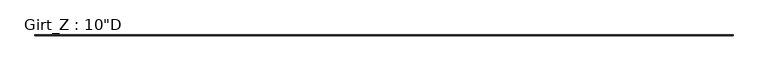
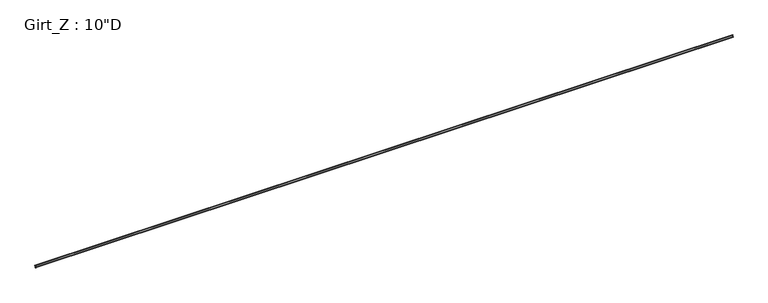
"""IFC4 building model written with IfcOpenShell, lengths in millimetres: beam geometry."""

import ifcopenshell
import ifcopenshell.guid

model = None  # the IFC model being written
_history = None  # IfcOwnerHistory: only IFC2X3 demands one
_inside = {}  # id of a spatial element -> (the spatial element, [elements in it])
_under = {}  # id of a project, library or spatial element -> (it, [spatial elements below it])
_declared = {}  # id of a project -> (the project, [libraries it declares])
_typed = {}  # id of a type object -> (the type object, [elements of that type])
_made_of = {}  # id of a material, layer set ... -> (it, [elements and type objects made of it])


def new_model(schema):
    """Start an empty IFC model of exactly this schema.

    Asked for "IFC4X3", IfcOpenShell would pick the latest addendum, in which some entities
    have other attributes; the version numbers below select the first issue.
    IFC2X3 requires an IfcOwnerHistory on every rooted entity: one is made here for all.
    """
    global model, _history
    if schema == "IFC4X3":
        model = ifcopenshell.file(schema_version=(4, 3, 0, 0))
    else:
        model = ifcopenshell.file(schema=schema)
    _inside.clear()
    _under.clear()
    _declared.clear()
    _typed.clear()
    _made_of.clear()
    _history = None
    if model.schema == "IFC2X3":
        org = make("IfcOrganization", Name="unknown")
        user = make(
            "IfcPersonAndOrganization",
            ThePerson=make("IfcPerson", FamilyName="unknown"),
            TheOrganization=org,
        )
        app = make(
            "IfcApplication",
            ApplicationDeveloper=org,
            Version="unknown",
            ApplicationFullName="unknown",
            ApplicationIdentifier="unknown",
        )
        _history = make(
            "IfcOwnerHistory",
            OwningUser=user,
            OwningApplication=app,
            ChangeAction="ADDED",
            CreationDate=0,
        )
    return model


def make(cls, **values):
    """One entity of the class cls with the attributes given. An attribute that is None is left unset."""
    return model.create_entity(
        cls, **{name: value for name, value in values.items() if value is not None}
    )


def rooted(cls, **values):
    """An entity with a GlobalId (a new one), such as an element, a storey or a relation."""
    return make(cls, GlobalId=ifcopenshell.guid.new(), OwnerHistory=_history, **values)


def si_unit(unit_type, name, prefix=None):
    """IfcSIUnit, for example si_unit("LENGTHUNIT", "METRE", prefix="MILLI")."""
    return make("IfcSIUnit", UnitType=unit_type, Prefix=prefix, Name=name)


def assignment(units):
    """IfcUnitAssignment: the units of a project."""
    return None if units is None else make("IfcUnitAssignment", Units=units)


def point(xyz):
    """IfcCartesianPoint."""
    return None if xyz is None else make("IfcCartesianPoint", Coordinates=xyz)


def direction(xyz):
    """IfcDirection."""
    return None if xyz is None else make("IfcDirection", DirectionRatios=xyz)


def frame(location, z_axis=None, x_axis=None):
    """IfcAxis2Placement3D, a coordinate frame: its origin and axes. An axis left out is left unset."""
    return make(
        "IfcAxis2Placement3D",
        Location=point(location),
        Axis=direction(z_axis),
        RefDirection=direction(x_axis),
    )


def frame_2d(location, x_axis=None):
    """IfcAxis2Placement2D, a coordinate frame in the plane: its origin and x axis."""
    return make(
        "IfcAxis2Placement2D", Location=point(location), RefDirection=direction(x_axis)
    )


def origin():
    """The frame at (0, 0, 0) with its axes left unset."""
    return frame((0.0, 0.0, 0.0))


def place(relative_to, where):
    """IfcLocalPlacement: puts the frame where relative to a parent placement (None: the world)."""
    return make(
        "IfcLocalPlacement", PlacementRelTo=relative_to, RelativePlacement=where
    )


def context(
    kind, dimensions, precision=None, world=None, true_north=None, identifier=None
):
    """IfcGeometricRepresentationContext, for example the 3D "Model" context."""
    return make(
        "IfcGeometricRepresentationContext",
        ContextIdentifier=identifier,
        ContextType=kind,
        CoordinateSpaceDimension=dimensions,
        Precision=precision,
        WorldCoordinateSystem=world,
        TrueNorth=true_north,
    )


def project(units=None, contexts=None):
    """IfcProject with its units and contexts."""
    return rooted(
        "IfcProject",
        Name="project",
        RepresentationContexts=contexts,
        UnitsInContext=assignment(units),
    )


def spatial(cls, under=None, at=None, **own):
    """A site, building, storey or space (cls), placed at a placement, below another one or the project."""
    s = rooted(cls, ObjectPlacement=at, **own)
    if under is not None:
        _under.setdefault(under.id(), (under, []))[1].append(s)
    return s


def polyline(points):
    """IfcPolyline through the points."""
    return make("IfcPolyline", Points=[point(p) for p in points])


def circle_curve(where, radius):
    """IfcCircle in the frame where."""
    return make("IfcCircle", Position=where, Radius=radius)


def trimmed(basis, trim1, trim2, sense, master):
    """IfcTrimmedCurve: the piece of a basis curve between two trims."""
    return make(
        "IfcTrimmedCurve",
        BasisCurve=basis,
        Trim1=trim1,
        Trim2=trim2,
        SenseAgreement=sense,
        MasterRepresentation=master,
    )


def segment(curve, same_sense, transition):
    """IfcCompositeCurveSegment."""
    return make(
        "IfcCompositeCurveSegment",
        Transition=transition,
        SameSense=same_sense,
        ParentCurve=curve,
    )


def composite_curve(segments, self_intersect=None):
    """IfcCompositeCurve: segments joined end to end."""
    return make("IfcCompositeCurve", Segments=segments, SelfIntersect=self_intersect)


def outline(outer, holes=None, kind="AREA"):
    """IfcArbitraryClosedProfileDef: a profile drawn as a closed curve; with holes, ...WithVoids."""
    if holes is None:
        return make("IfcArbitraryClosedProfileDef", ProfileType=kind, OuterCurve=outer)
    return make(
        "IfcArbitraryProfileDefWithVoids",
        ProfileType=kind,
        OuterCurve=outer,
        InnerCurves=holes,
    )


def extrude(swept, where, along, depth):
    """IfcExtrudedAreaSolid: the profile swept, set in the frame where, extruded along a direction by depth."""
    return make(
        "IfcExtrudedAreaSolid",
        SweptArea=swept,
        Position=where,
        ExtrudedDirection=direction(along),
        Depth=depth,
    )


def shape(context_of_items, identifier, shape_type, items):
    """IfcShapeRepresentation: the items that make up one representation, for example the "Body"."""
    return make(
        "IfcShapeRepresentation",
        ContextOfItems=context_of_items,
        RepresentationIdentifier=identifier,
        RepresentationType=shape_type,
        Items=items,
    )


def source(mapping_origin, context_of_items, identifier, shape_type, items):
    """IfcRepresentationMap: a shape defined once, which mapped items show again and again."""
    return make(
        "IfcRepresentationMap",
        MappingOrigin=mapping_origin,
        MappedRepresentation=shape(context_of_items, identifier, shape_type, items),
    )


def transform(
    local_origin,
    x_axis=None,
    y_axis=None,
    z_axis=None,
    scale=None,
    scale2=None,
    scale3=None,
    uniform=True,
):
    """IfcCartesianTransformationOperator3D, or its non-uniform kind. x_axis, y_axis, z_axis: its Axis1, 2, 3."""
    if uniform:
        return make(
            "IfcCartesianTransformationOperator3D",
            Axis1=direction(x_axis),
            Axis2=direction(y_axis),
            LocalOrigin=point(local_origin),
            Scale=scale,
            Axis3=direction(z_axis),
        )
    return make(
        "IfcCartesianTransformationOperator3DnonUniform",
        Axis1=direction(x_axis),
        Axis2=direction(y_axis),
        LocalOrigin=point(local_origin),
        Scale=scale,
        Axis3=direction(z_axis),
        Scale2=scale2,
        Scale3=scale3,
    )


def mapped(mapping_source, mapping_target):
    """IfcMappedItem: shows the shape of a source again, moved by a transform."""
    return make(
        "IfcMappedItem", MappingSource=mapping_source, MappingTarget=mapping_target
    )


def made_of(thing, what):
    """Note that an element or type object is made of a material, layer set ...; save() writes the relation."""
    if what is not None:
        _made_of.setdefault(what.id(), (what, []))[1].append(thing)
    return thing


def element(
    cls,
    number,
    at=None,
    inside=None,
    cuts=None,
    type_object=None,
    material=None,
    context=None,
    identifier="Body",
    shape_type=None,
    held_by="IfcProductDefinitionShape",
    body=None,
    shapes=None,
    **own,
):
    """One element of the class cls, such as IfcWall. Its Tag is "e" and its number.

    at: its placement. inside: the storey or other place that contains it. cuts: it is an
    opening in that element (IfcRelVoidsElement). A single representation is given by context,
    identifier, shape_type and body (its items); several are given by shapes. held_by: the class
    of the entity that holds the representations. save() writes the other relations.
    """
    e = rooted(cls, Tag="e%d" % number, ObjectPlacement=at, **own)
    if body is not None:
        shapes = [shape(context, identifier, shape_type, body)]
    if shapes is not None:
        e.Representation = make(held_by, Representations=shapes)
    if inside is not None:
        _inside.setdefault(inside.id(), (inside, []))[1].append(e)
    if cuts is not None:
        rooted(
            "IfcRelVoidsElement", RelatingBuildingElement=cuts, RelatedOpeningElement=e
        )
    if type_object is not None:
        _typed.setdefault(type_object.id(), (type_object, []))[1].append(e)
    return made_of(e, material)


def aggregate(whole, parts):
    """IfcRelAggregates: a whole, such as a stair, and the parts it consists of."""
    return rooted("IfcRelAggregates", RelatingObject=whole, RelatedObjects=parts)


def save(model, path):
    """Write the relations noted so far, then the file.

    IfcRelAggregates (storeys below a building ...), IfcRelContainedInSpatialStructure (elements
    in a storey), IfcRelDefinesByType, IfcRelAssociatesMaterial and IfcRelDeclares: one each for
    every whole, place, type object, material and project.
    """
    for whole, parts in _under.values():
        aggregate(whole, parts)
    for where, things in _inside.values():
        rooted(
            "IfcRelContainedInSpatialStructure",
            RelatedElements=things,
            RelatingStructure=where,
        )
    for kind, things in _typed.values():
        rooted("IfcRelDefinesByType", RelatedObjects=things, RelatingType=kind)
    for what, things in _made_of.values():
        rooted("IfcRelAssociatesMaterial", RelatedObjects=things, RelatingMaterial=what)
    for by, libraries in _declared.values():
        rooted("IfcRelDeclares", RelatingContext=by, RelatedDefinitions=libraries)
    model.write(path)


def beam_6747da0e(model_context):
    return source(origin(), model_context, "Body", "SweptSolid", [
        extrude(outline(composite_curve([segment(polyline([(63.5, 127.0), (75.745104, 112.4068534), (73.6169367, 110.621109), (62.204539, 124.221875), (3.3005807, 124.221875)]), True, "CONTINUOUS"), segment(trimmed(circle_curve(frame_2d((3.3741066, 122.2381931)), 1.9850441), [point((3.3005807, 124.221875))], [point((1.3890625, 122.2381931))], True, "CARTESIAN"), True, "CONTINUOUS"), segment(polyline([(1.3890625, 122.2381931), (1.3890625, -122.2375)]), True, "CONTINUOUS"), segment(trimmed(circle_curve(frame_2d((-3.3734375, -122.2375)), 4.7625), [point((1.3890625, -122.2375))], [point((-3.3734375, -127.0))], False, "CARTESIAN"), True, "CONTINUOUS"), segment(polyline([(-3.3734375, -127.0), (-63.5, -127.0), (-75.745104, -112.4068534), (-73.6169367, -110.621109), (-62.204539, -124.221875), (-3.2694106, -124.221875)]), True, "CONTINUOUS"), segment(trimmed(circle_curve(frame_2d((-3.3748024, -122.2389339)), 1.9857399), [point((-3.2694106, -124.221875))], [point((-1.3890625, -122.2389339))], True, "CARTESIAN"), True, "CONTINUOUS"), segment(polyline([(-1.3890625, -122.2389339), (-1.3890625, 122.2375)]), True, "CONTINUOUS"), segment(trimmed(circle_curve(frame_2d((3.3734375, 122.2375)), 4.7625), [point((-1.3890625, 122.2375))], [point((3.3734375, 127.0))], False, "CARTESIAN"), True, "CONTINUOUS"), segment(polyline([(3.3734375, 127.0), (63.5, 127.0)]), True, "CONTINUOUS")], self_intersect=False)), frame((-52273.2, 0.0, 0.0), z_axis=(1.0, 0.0, 0.0), x_axis=(0.0, 1.0, 0.0)), (0.0, 0.0, 1.0), 104546.4),
    ])


if __name__ == "__main__":
    model = new_model("IFC4")
    model_context = context("Model", 3, world=origin())
    ifc_project = project(units=[si_unit("LENGTHUNIT", "METRE", prefix="MILLI")], contexts=[model_context])
    site = spatial("IfcSite", under=ifc_project)
    building = spatial("IfcBuilding", under=site)
    placement = place(None, origin())
    beam_shape = beam_6747da0e(model_context)
    element("IfcBeam", 1, ObjectType="Girt_Z : 10\"D", at=placement, inside=building, context=model_context, shape_type="MappedRepresentation", body=[
        mapped(beam_shape, transform((0.0, 0.0, 0.0), x_axis=(1.0, 0.0, 0.0), y_axis=(0.0, 1.0, 0.0), z_axis=(0.0, 0.0, 1.0))),
    ])
    save(model, "model.ifc")

# Revit data of these elements
# Type "Girt_Z : 10\"D"
#   Web_Thickness = 0' - 0 7/64"
#   Length [instance default] = 10' - 0"
#   Leg_1 = 0' - 2 1/2"
#   Height = 0' - 10"
